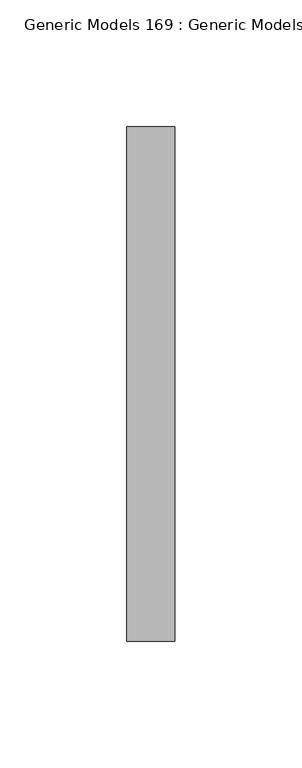
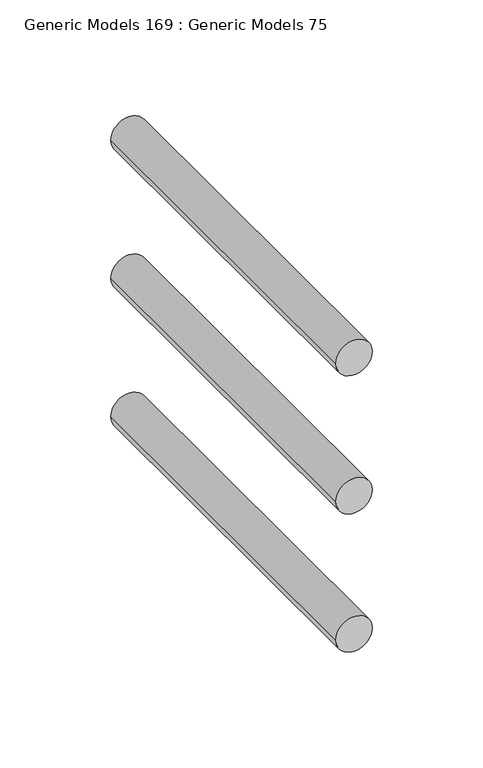
"""IFC4 building model written with IfcOpenShell, lengths in millimetres: proxy geometry, Generic Models 169 : Generic Models 75."""

from ifc_helpers import new_model, si_unit, point, frame, frame_2d, origin, place, context, project, spatial, circle_curve, trimmed, segment, composite_curve, outline, extrude, source, transform, mapped, element, save


def generic_models_169_generic_models_75_3ab922b0(model_context):
    return source(origin(), model_context, "Body", "SweptSolid", [
        extrude(outline(composite_curve([segment(trimmed(circle_curve(frame_2d((271765.7125, 31705.5346032)), 9.525), [point((271765.7125, 31696.0096032))], [point((271765.7125, 31715.0596032))], False, "CARTESIAN"), True, "CONTINUOUS"), segment(trimmed(circle_curve(frame_2d((271765.7125, 31705.5346032)), 9.525), [point((271765.7125, 31715.0596032))], [point((271765.7125, 31696.0096032))], False, "CARTESIAN"), True, "CONTINUOUS")], self_intersect=False)), frame((0.0, 30672.7406612, 0.0), z_axis=(0.0, 1.0, 0.0), x_axis=(0.0, 0.0, 1.0)), (0.0, 0.0, 1.0), 203.2),
        extrude(outline(composite_curve([segment(trimmed(circle_curve(frame_2d((271689.5125, 31705.5346032)), 9.525), [point((271689.5125, 31696.0096032))], [point((271689.5125, 31715.0596032))], False, "CARTESIAN"), True, "CONTINUOUS"), segment(trimmed(circle_curve(frame_2d((271689.5125, 31705.5346032)), 9.525), [point((271689.5125, 31715.0596032))], [point((271689.5125, 31696.0096032))], False, "CARTESIAN"), True, "CONTINUOUS")], self_intersect=False)), frame((0.0, 30672.7406612, 0.0), z_axis=(0.0, 1.0, 0.0), x_axis=(0.0, 0.0, 1.0)), (0.0, 0.0, 1.0), 203.2),
        extrude(outline(composite_curve([segment(trimmed(circle_curve(frame_2d((271841.9125, 31705.5346032)), 9.525), [point((271841.9125, 31696.0096032))], [point((271841.9125, 31715.0596032))], False, "CARTESIAN"), True, "CONTINUOUS"), segment(trimmed(circle_curve(frame_2d((271841.9125, 31705.5346032)), 9.525), [point((271841.9125, 31715.0596032))], [point((271841.9125, 31696.0096032))], False, "CARTESIAN"), True, "CONTINUOUS")], self_intersect=False)), frame((0.0, 30672.7406612, 0.0), z_axis=(0.0, 1.0, 0.0), x_axis=(0.0, 0.0, 1.0)), (0.0, 0.0, 1.0), 203.2),
    ])


if __name__ == "__main__":
    model = new_model("IFC4")
    model_context = context("Model", 3, world=origin())
    ifc_project = project(units=[si_unit("LENGTHUNIT", "METRE", prefix="MILLI")], contexts=[model_context])
    site = spatial("IfcSite", under=ifc_project)
    building = spatial("IfcBuilding", under=site)
    placement = place(None, origin())
    generic_models_169_generic_models_75_shape = generic_models_169_generic_models_75_3ab922b0(model_context)
    element("IfcBuildingElementProxy", 1, Name="Generic Models 169 : Generic Models 75", ObjectType="Generic Models 169 : Generic Models 75", at=placement, inside=building, context=model_context, shape_type="MappedRepresentation", body=[
        mapped(generic_models_169_generic_models_75_shape, transform((0.0, 0.0, 0.0), x_axis=(1.0, 0.0, 0.0), y_axis=(0.0, 1.0, 0.0), z_axis=(0.0, 0.0, 1.0))),
    ])
    save(model, "model.ifc")
